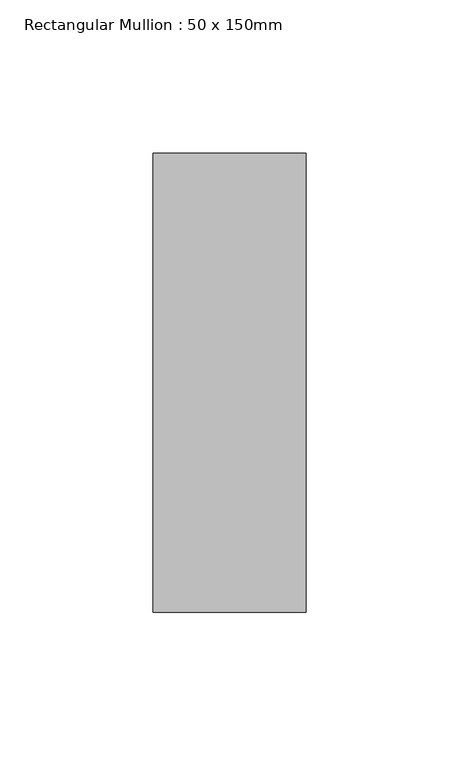
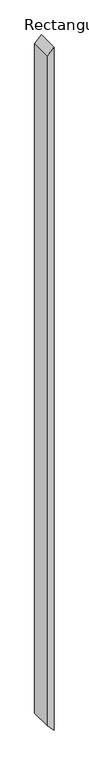
"""IFC4 building model written with IfcOpenShell, lengths in millimetres: member geometry, Rectangular Mullion : 50 x 150mm."""

from ifc_helpers import new_model, si_unit, frame, origin, place, context, project, spatial, polyline, outline, extrude, source, transform, mapped, element, save


def rectangular_mullion_50_x_150mm_0be3d6d3(model_context):
    return source(origin(), model_context, "Body", "SweptSolid", [
        extrude(outline(polyline([(0.0, 0.0), (-50.0, -50.0), (-5062.5032273, -50.0), (-5115.611673, 0.0), (0.0, 0.0)])), frame((0.0, -75.0, 0.0), z_axis=(0.0, 1.0, 0.0), x_axis=(0.0, 0.0, 1.0)), (0.0, 0.0, 1.0), 150.0),
    ])


if __name__ == "__main__":
    model = new_model("IFC4")
    model_context = context("Model", 3, world=origin())
    ifc_project = project(units=[si_unit("LENGTHUNIT", "METRE", prefix="MILLI")], contexts=[model_context])
    site = spatial("IfcSite", under=ifc_project)
    building = spatial("IfcBuilding", under=site)
    placement = place(None, origin())
    rectangular_mullion_50_x_150mm_shape = rectangular_mullion_50_x_150mm_0be3d6d3(model_context)
    element("IfcMember", 1, ObjectType="Rectangular Mullion : 50 x 150mm", at=placement, inside=building, context=model_context, shape_type="MappedRepresentation", body=[
        mapped(rectangular_mullion_50_x_150mm_shape, transform((0.0, 0.0, 0.0), x_axis=(1.0, 0.0, 0.0), y_axis=(0.0, 1.0, 0.0), z_axis=(0.0, 0.0, 1.0))),
    ])
    save(model, "model.ifc")

# Revit data of these elements
# Type "Rectangular Mullion : 50 x 150mm"
#   built-in parameter 1007304 = 0.492126 (stored number, unit not read)
#   built-in parameter 1007301 = 0.082021 (stored number, unit not read)
#   built-in parameter 1007300 = 0.082021 (stored number, unit not read)
# Element 1 (IfcMember, "Rectangular Mullion : 50 x 150mm")
#   Materials on its faces: "Metal - Aluminium"
# Materials
#   "Metal - Aluminium": class "Metal", colour RGB 247 247 247, transparency 0
